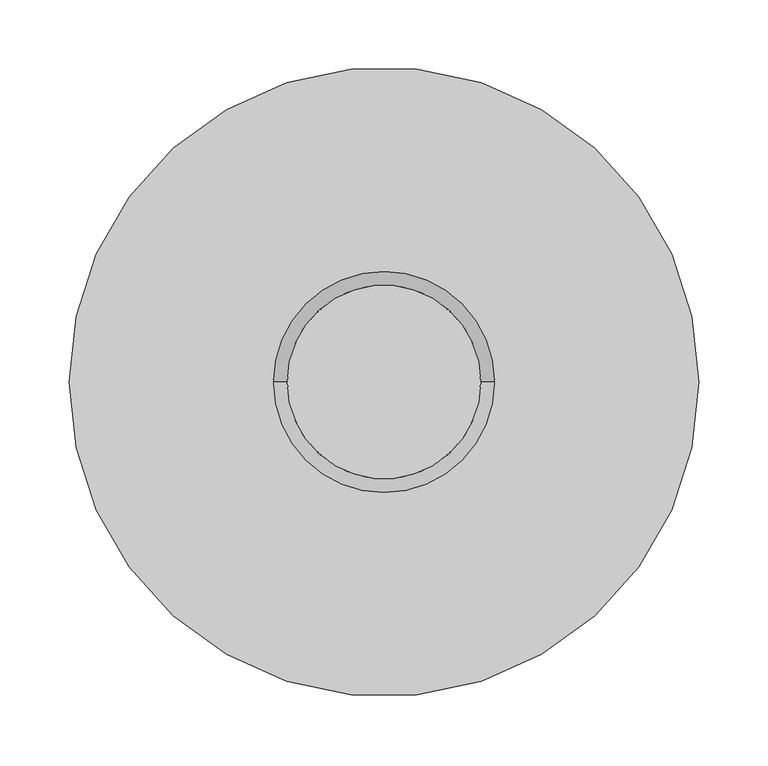
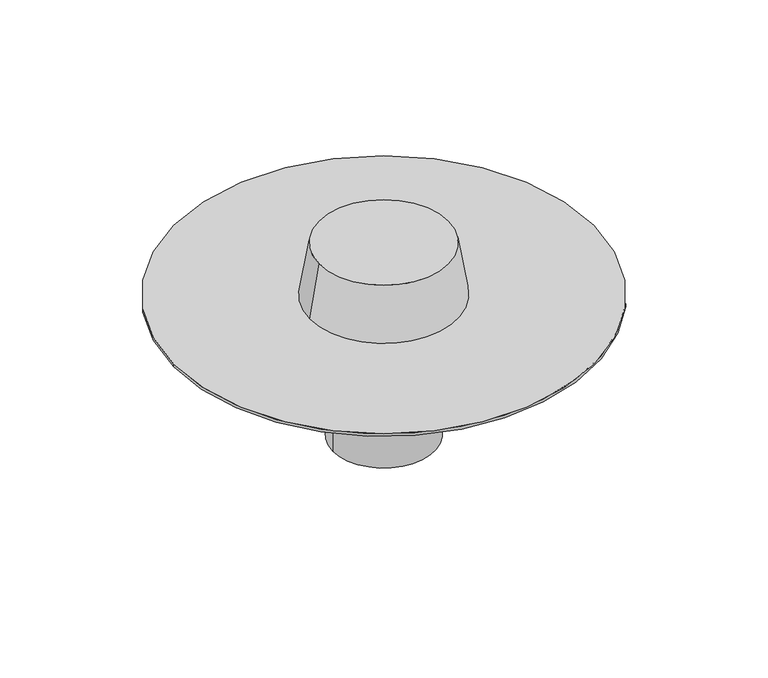
"""IFC4 building model written with IfcOpenShell, lengths in millimetres: proxy geometry, TN_Воронка ТехноНИКОЛЬ ВБ : ВоронкаТехноНИКОЛЬ ВБ, 110х160."""

import ifcopenshell
import ifcopenshell.guid

model = None  # the IFC model being written
_history = None  # IfcOwnerHistory: only IFC2X3 demands one
_inside = {}  # id of a spatial element -> (the spatial element, [elements in it])
_under = {}  # id of a project, library or spatial element -> (it, [spatial elements below it])
_declared = {}  # id of a project -> (the project, [libraries it declares])
_typed = {}  # id of a type object -> (the type object, [elements of that type])
_made_of = {}  # id of a material, layer set ... -> (it, [elements and type objects made of it])


def new_model(schema):
    """Start an empty IFC model of exactly this schema.

    Asked for "IFC4X3", IfcOpenShell would pick the latest addendum, in which some entities
    have other attributes; the version numbers below select the first issue.
    IFC2X3 requires an IfcOwnerHistory on every rooted entity: one is made here for all.
    """
    global model, _history
    if schema == "IFC4X3":
        model = ifcopenshell.file(schema_version=(4, 3, 0, 0))
    else:
        model = ifcopenshell.file(schema=schema)
    _inside.clear()
    _under.clear()
    _declared.clear()
    _typed.clear()
    _made_of.clear()
    _history = None
    if model.schema == "IFC2X3":
        org = make("IfcOrganization", Name="unknown")
        user = make(
            "IfcPersonAndOrganization",
            ThePerson=make("IfcPerson", FamilyName="unknown"),
            TheOrganization=org,
        )
        app = make(
            "IfcApplication",
            ApplicationDeveloper=org,
            Version="unknown",
            ApplicationFullName="unknown",
            ApplicationIdentifier="unknown",
        )
        _history = make(
            "IfcOwnerHistory",
            OwningUser=user,
            OwningApplication=app,
            ChangeAction="ADDED",
            CreationDate=0,
        )
    return model


def make(cls, **values):
    """One entity of the class cls with the attributes given. An attribute that is None is left unset."""
    return model.create_entity(
        cls, **{name: value for name, value in values.items() if value is not None}
    )


def rooted(cls, **values):
    """An entity with a GlobalId (a new one), such as an element, a storey or a relation."""
    return make(cls, GlobalId=ifcopenshell.guid.new(), OwnerHistory=_history, **values)


def si_unit(unit_type, name, prefix=None):
    """IfcSIUnit, for example si_unit("LENGTHUNIT", "METRE", prefix="MILLI")."""
    return make("IfcSIUnit", UnitType=unit_type, Prefix=prefix, Name=name)


def assignment(units):
    """IfcUnitAssignment: the units of a project."""
    return None if units is None else make("IfcUnitAssignment", Units=units)


def point(xyz):
    """IfcCartesianPoint."""
    return None if xyz is None else make("IfcCartesianPoint", Coordinates=xyz)


def direction(xyz):
    """IfcDirection."""
    return None if xyz is None else make("IfcDirection", DirectionRatios=xyz)


def frame(location, z_axis=None, x_axis=None):
    """IfcAxis2Placement3D, a coordinate frame: its origin and axes. An axis left out is left unset."""
    return make(
        "IfcAxis2Placement3D",
        Location=point(location),
        Axis=direction(z_axis),
        RefDirection=direction(x_axis),
    )


def frame_2d(location, x_axis=None):
    """IfcAxis2Placement2D, a coordinate frame in the plane: its origin and x axis."""
    return make(
        "IfcAxis2Placement2D", Location=point(location), RefDirection=direction(x_axis)
    )


def origin():
    """The frame at (0, 0, 0) with its axes left unset."""
    return frame((0.0, 0.0, 0.0))


def origin_2d():
    """The frame at (0, 0) in the plane with its x axis left unset."""
    return frame_2d((0.0, 0.0))


def place(relative_to, where):
    """IfcLocalPlacement: puts the frame where relative to a parent placement (None: the world)."""
    return make(
        "IfcLocalPlacement", PlacementRelTo=relative_to, RelativePlacement=where
    )


def context(
    kind, dimensions, precision=None, world=None, true_north=None, identifier=None
):
    """IfcGeometricRepresentationContext, for example the 3D "Model" context."""
    return make(
        "IfcGeometricRepresentationContext",
        ContextIdentifier=identifier,
        ContextType=kind,
        CoordinateSpaceDimension=dimensions,
        Precision=precision,
        WorldCoordinateSystem=world,
        TrueNorth=true_north,
    )


def project(units=None, contexts=None):
    """IfcProject with its units and contexts."""
    return rooted(
        "IfcProject",
        Name="project",
        RepresentationContexts=contexts,
        UnitsInContext=assignment(units),
    )


def spatial(cls, under=None, at=None, **own):
    """A site, building, storey or space (cls), placed at a placement, below another one or the project."""
    s = rooted(cls, ObjectPlacement=at, **own)
    if under is not None:
        _under.setdefault(under.id(), (under, []))[1].append(s)
    return s


def polyline(points):
    """IfcPolyline through the points."""
    return make("IfcPolyline", Points=[point(p) for p in points])


def circle_curve(where, radius):
    """IfcCircle in the frame where."""
    return make("IfcCircle", Position=where, Radius=radius)


def trimmed(basis, trim1, trim2, sense, master):
    """IfcTrimmedCurve: the piece of a basis curve between two trims."""
    return make(
        "IfcTrimmedCurve",
        BasisCurve=basis,
        Trim1=trim1,
        Trim2=trim2,
        SenseAgreement=sense,
        MasterRepresentation=master,
    )


def segment(curve, same_sense, transition):
    """IfcCompositeCurveSegment."""
    return make(
        "IfcCompositeCurveSegment",
        Transition=transition,
        SameSense=same_sense,
        ParentCurve=curve,
    )


def composite_curve(segments, self_intersect=None):
    """IfcCompositeCurve: segments joined end to end."""
    return make("IfcCompositeCurve", Segments=segments, SelfIntersect=self_intersect)


def outline(outer, holes=None, kind="AREA"):
    """IfcArbitraryClosedProfileDef: a profile drawn as a closed curve; with holes, ...WithVoids."""
    if holes is None:
        return make("IfcArbitraryClosedProfileDef", ProfileType=kind, OuterCurve=outer)
    return make(
        "IfcArbitraryProfileDefWithVoids",
        ProfileType=kind,
        OuterCurve=outer,
        InnerCurves=holes,
    )


def extrude(swept, where, along, depth):
    """IfcExtrudedAreaSolid: the profile swept, set in the frame where, extruded along a direction by depth."""
    return make(
        "IfcExtrudedAreaSolid",
        SweptArea=swept,
        Position=where,
        ExtrudedDirection=direction(along),
        Depth=depth,
    )


def shape(context_of_items, identifier, shape_type, items):
    """IfcShapeRepresentation: the items that make up one representation, for example the "Body"."""
    return make(
        "IfcShapeRepresentation",
        ContextOfItems=context_of_items,
        RepresentationIdentifier=identifier,
        RepresentationType=shape_type,
        Items=items,
    )


def source(mapping_origin, context_of_items, identifier, shape_type, items):
    """IfcRepresentationMap: a shape defined once, which mapped items show again and again."""
    return make(
        "IfcRepresentationMap",
        MappingOrigin=mapping_origin,
        MappedRepresentation=shape(context_of_items, identifier, shape_type, items),
    )


def transform(
    local_origin,
    x_axis=None,
    y_axis=None,
    z_axis=None,
    scale=None,
    scale2=None,
    scale3=None,
    uniform=True,
):
    """IfcCartesianTransformationOperator3D, or its non-uniform kind. x_axis, y_axis, z_axis: its Axis1, 2, 3."""
    if uniform:
        return make(
            "IfcCartesianTransformationOperator3D",
            Axis1=direction(x_axis),
            Axis2=direction(y_axis),
            LocalOrigin=point(local_origin),
            Scale=scale,
            Axis3=direction(z_axis),
        )
    return make(
        "IfcCartesianTransformationOperator3DnonUniform",
        Axis1=direction(x_axis),
        Axis2=direction(y_axis),
        LocalOrigin=point(local_origin),
        Scale=scale,
        Axis3=direction(z_axis),
        Scale2=scale2,
        Scale3=scale3,
    )


def mapped(mapping_source, mapping_target):
    """IfcMappedItem: shows the shape of a source again, moved by a transform."""
    return make(
        "IfcMappedItem", MappingSource=mapping_source, MappingTarget=mapping_target
    )


def made_of(thing, what):
    """Note that an element or type object is made of a material, layer set ...; save() writes the relation."""
    if what is not None:
        _made_of.setdefault(what.id(), (what, []))[1].append(thing)
    return thing


def element(
    cls,
    number,
    at=None,
    inside=None,
    cuts=None,
    type_object=None,
    material=None,
    context=None,
    identifier="Body",
    shape_type=None,
    held_by="IfcProductDefinitionShape",
    body=None,
    shapes=None,
    **own,
):
    """One element of the class cls, such as IfcWall. Its Tag is "e" and its number.

    at: its placement. inside: the storey or other place that contains it. cuts: it is an
    opening in that element (IfcRelVoidsElement). A single representation is given by context,
    identifier, shape_type and body (its items); several are given by shapes. held_by: the class
    of the entity that holds the representations. save() writes the other relations.
    """
    e = rooted(cls, Tag="e%d" % number, ObjectPlacement=at, **own)
    if body is not None:
        shapes = [shape(context, identifier, shape_type, body)]
    if shapes is not None:
        e.Representation = make(held_by, Representations=shapes)
    if inside is not None:
        _inside.setdefault(inside.id(), (inside, []))[1].append(e)
    if cuts is not None:
        rooted(
            "IfcRelVoidsElement", RelatingBuildingElement=cuts, RelatedOpeningElement=e
        )
    if type_object is not None:
        _typed.setdefault(type_object.id(), (type_object, []))[1].append(e)
    return made_of(e, material)


def aggregate(whole, parts):
    """IfcRelAggregates: a whole, such as a stair, and the parts it consists of."""
    return rooted("IfcRelAggregates", RelatingObject=whole, RelatedObjects=parts)


def save(model, path):
    """Write the relations noted so far, then the file.

    IfcRelAggregates (storeys below a building ...), IfcRelContainedInSpatialStructure (elements
    in a storey), IfcRelDefinesByType, IfcRelAssociatesMaterial and IfcRelDeclares: one each for
    every whole, place, type object, material and project.
    """
    for whole, parts in _under.values():
        aggregate(whole, parts)
    for where, things in _inside.values():
        rooted(
            "IfcRelContainedInSpatialStructure",
            RelatedElements=things,
            RelatingStructure=where,
        )
    for kind, things in _typed.values():
        rooted("IfcRelDefinesByType", RelatedObjects=things, RelatingType=kind)
    for what, things in _made_of.values():
        rooted("IfcRelAssociatesMaterial", RelatedObjects=things, RelatingMaterial=what)
    for by, libraries in _declared.values():
        rooted("IfcRelDeclares", RelatingContext=by, RelatedDefinitions=libraries)
    model.write(path)


def plane_surface(at):
    """IfcPlane: the flat surface through the origin of the frame at, square to its z axis."""
    return make("IfcPlane", Position=at)


def revolved_surface(curve, axis_point, axis_direction):
    """IfcSurfaceOfRevolution: the curve turned about the line through axis_point along axis_direction."""
    return make(
        "IfcSurfaceOfRevolution",
        SweptCurve=make("IfcArbitraryOpenProfileDef", ProfileType="CURVE", Curve=curve),
        AxisPosition=make("IfcAxis1Placement", Location=point(axis_point), Axis=direction(axis_direction)),
    )


def advanced_brep(points, edges, surfaces, faces):
    """IfcAdvancedBrep: a solid bounded by faces that lie on surfaces and meet in shared edges.

    An edge is (start, end): straight between two places in points (the first is 0);
    or (start, end, curve); or (start, end, curve, False) where it runs against its curve.
    A face is (place in surfaces, loops), or (place, loops, False) where it looks against
    its surface's normal. A loop lists edges by number (the first is 1), with a minus sign
    where the edge is run from its end to its start. The first loop is the outer one.
    """
    corners = [point(p) for p in points]
    vertices = [make("IfcVertexPoint", VertexGeometry=c) for c in corners]
    made = []
    for start, end, *more in edges:
        made.append(
            make(
                "IfcEdgeCurve",
                EdgeStart=vertices[start],
                EdgeEnd=vertices[end],
                EdgeGeometry=more[0] if more else make("IfcPolyline", Points=[corners[start], corners[end]]),
                SameSense=more[1] if len(more) > 1 else True,
            )
        )
    hull = []
    for where, loops, *sense in faces:
        bounds = []
        for j, loop in enumerate(loops):
            ring = [make("IfcOrientedEdge", EdgeElement=made[abs(k) - 1], Orientation=k > 0) for k in loop]
            bounds.append(
                make(
                    "IfcFaceOuterBound" if j == 0 else "IfcFaceBound",
                    Bound=make("IfcEdgeLoop", EdgeList=ring),
                    Orientation=True,
                )
            )
        hull.append(make("IfcAdvancedFace", Bounds=bounds, FaceSurface=surfaces[where], SameSense=sense[0] if sense else True))
    return make("IfcAdvancedBrep", Outer=make("IfcClosedShell", CfsFaces=hull))


def specialty_equipment_725ca240(model_context):
    return source(origin(), model_context, "Body", "SolidModel", [
        advanced_brep(
        [(70.0, 0.0, -85.0), (-70.0, 0.0, -85.0), (55.0, 0.0, -120.0), (-55.0, 0.0, -120.0)],
        [
            (0, 1, circle_curve(frame((0.0, 0.0, -85.0), z_axis=(0.0, 0.0, 1.0), x_axis=(1.0, 0.0, 0.0)), 70.0)),
            (1, 0, circle_curve(frame((0.0, 0.0, -85.0), z_axis=(0.0, 0.0, 1.0), x_axis=(-1.0, 0.0, 0.0)), 70.0)),
            (2, 3, circle_curve(frame((0.0, 0.0, -120.0), z_axis=(0.0, 0.0, -1.0), x_axis=(-1.0, 0.0, 0.0)), 55.0)),
            (3, 2, circle_curve(frame((0.0, 0.0, -120.0), z_axis=(0.0, 0.0, -1.0), x_axis=(1.0, 0.0, 0.0)), 55.0)),
            (3, 1),
            (0, 2),
        ],
        [
            plane_surface(frame((0.0, 0.0, -85.0), z_axis=(0.0, 0.0, 1.0), x_axis=(0.0, 1.0, 0.0))),
            plane_surface(frame((0.0, 0.0, -120.0), z_axis=(0.0, 0.0, -1.0), x_axis=(0.0, 1.0, 0.0))),
            revolved_surface(polyline([(-54.999999996938776, 0.0, -120.0), (-70.0, 0.0, -85.0)]), (0.0, 0.0, -248.3333333), (0.0, 0.0, 1.0)),
            revolved_surface(polyline([(54.999999996938776, 0.0, -120.0), (70.0, 0.0, -85.0)]), (0.0, 0.0, -248.3333333), (0.0, 0.0, 1.0)),
        ],
        [
            (0, [[1, 2]]),
            (1, [[3, 4]]),
            (2, [[-4, 5, -1, 6]]),
            (3, [[-3, -6, -2, -5]]),
        ],
    ),
        extrude(outline(composite_curve([segment(trimmed(circle_curve(origin_2d(), 70.0), [point((-70.0, 0.0))], [point((70.0, 0.0))], False, "CARTESIAN"), True, "CONTINUOUS"), segment(trimmed(circle_curve(origin_2d(), 70.0), [point((70.0, 0.0))], [point((-70.0, 0.0))], False, "CARTESIAN"), True, "CONTINUOUS")], self_intersect=False)), frame((0.0, 0.0, -85.0), z_axis=(0.0, 0.0, 1.0), x_axis=(1.0, 0.0, 0.0)), (0.0, 0.0, 1.0), 82.0),
        extrude(outline(composite_curve([segment(trimmed(circle_curve(origin_2d(), 55.0), [point((55.0, 0.0))], [point((-55.0, 0.0))], False, "CARTESIAN"), True, "CONTINUOUS"), segment(trimmed(circle_curve(origin_2d(), 55.0), [point((-55.0, 0.0))], [point((55.0, 0.0))], False, "CARTESIAN"), True, "CONTINUOUS")], self_intersect=False)), frame((0.0, 0.0, -160.0), z_axis=(0.0, 0.0, 1.0), x_axis=(1.0, 0.0, 0.0)), (0.0, 0.0, 1.0), 40.0),
        extrude(outline(composite_curve([segment(trimmed(circle_curve(origin_2d(), 227.5), [point((-227.5, 0.0))], [point((227.5, 0.0))], False, "CARTESIAN"), True, "CONTINUOUS"), segment(trimmed(circle_curve(origin_2d(), 227.5), [point((227.5, 0.0))], [point((-227.5, 0.0))], False, "CARTESIAN"), True, "CONTINUOUS")], self_intersect=False)), frame((0.0, 0.0, -3.0), z_axis=(0.0, 0.0, 1.0), x_axis=(1.0, 0.0, 0.0)), (0.0, 0.0, 1.0), 3.0),
        advanced_brep(
        [(-70.0, 0.0, 60.0), (70.0, 0.0, 60.0), (-80.0, 0.0, 0.0), (80.0, 0.0, 0.0)],
        [
            (0, 1, circle_curve(frame((0.0, 0.0, 60.0), z_axis=(0.0, 0.0, 1.0), x_axis=(-1.0, 0.0, 0.0)), 70.0)),
            (1, 0, circle_curve(frame((0.0, 0.0, 60.0), z_axis=(0.0, 0.0, 1.0), x_axis=(1.0, 0.0, 0.0)), 70.0)),
            (2, 3, circle_curve(frame((0.0, 0.0, 0.0), z_axis=(0.0, 0.0, -1.0), x_axis=(1.0, 0.0, 0.0)), 80.0)),
            (3, 2, circle_curve(frame((0.0, 0.0, 0.0), z_axis=(0.0, 0.0, -1.0), x_axis=(-1.0, 0.0, 0.0)), 80.0)),
            (3, 1),
            (0, 2),
        ],
        [
            plane_surface(frame((0.0, 0.0, 60.0), z_axis=(0.0, 0.0, 1.0), x_axis=(0.0, -1.0, 0.0))),
            plane_surface(frame((0.0, 0.0, 0.0), z_axis=(0.0, 0.0, -1.0), x_axis=(0.0, -1.0, 0.0))),
            revolved_surface(polyline([(-70.0, 0.0, 60.0), (-80.0, 0.0, 0.0)]), (0.0, 0.0, 480.0), (0.0, 0.0, -1.0)),
            revolved_surface(polyline([(70.0, 0.0, 60.0), (80.0, 0.0, 0.0)]), (0.0, 0.0, 480.0), (0.0, 0.0, -1.0)),
        ],
        [
            (0, [[1, 2]]),
            (1, [[3, 4]]),
            (2, [[-4, 5, -1, 6]]),
            (3, [[-3, -6, -2, -5]]),
        ],
    ),
    ])


if __name__ == "__main__":
    model = new_model("IFC4")
    model_context = context("Model", 3, world=origin())
    ifc_project = project(units=[si_unit("LENGTHUNIT", "METRE", prefix="MILLI")], contexts=[model_context])
    site = spatial("IfcSite", under=ifc_project)
    building = spatial("IfcBuilding", under=site)
    placement = place(None, origin())
    specialty_equipment_shape = specialty_equipment_725ca240(model_context)
    element("IfcBuildingElementProxy", 1, Name="TN_Воронка ТехноНИКОЛЬ ВБ : ВоронкаТехноНИКОЛЬ ВБ, 110х160", ObjectType="TN_Воронка ТехноНИКОЛЬ ВБ : ВоронкаТехноНИКОЛЬ ВБ, 110х160", at=placement, inside=building, context=model_context, shape_type="MappedRepresentation", body=[
        mapped(specialty_equipment_shape, transform((0.0, 0.0, 0.0), x_axis=(1.0, 0.0, 0.0), y_axis=(0.0, 1.0, 0.0), z_axis=(0.0, 0.0, 1.0))),
    ])
    save(model, "model.ifc")

# Revit data of these elements
# Type "TN_Воронка ТехноНИКОЛЬ ВБ : ВоронкаТехноНИКОЛЬ ВБ, 110х160"
#   ADSK_Группирование = "Комплектующие и воронки"
#   Description = "Воронка ВБ используется при ремонте и строительстве зданий и сооружений и предназначена для\nудаления дождевой воды с плоских кровель. Применяется в кровлях из битумных и битумно-полимерных\nрулонных и мастичных материалов с внутренним водостоком. Рекомендуется устанавливать одну\nворонку примерно на каждые 250 м2 кровли, но требуется не менее двух водоотводящих систем на\nкровлю ограниченную парапетами. Пропуская способность 7,8 л/сек."
#   Manufacturer = "ТехноНИКОЛЬ"
#   URL = "http://nav.tn.ru/upload/iblock/67f/67f1681bb0d078f2e8af03b9528f2af6.pdf"
#   ADSK_Примечание = ""
#   ADSK_Обозначение = "ТехноНИКОЛЬ"
#   ADSK_Наименование = "Воронка ТехноНИКОЛЬ ВБ, 110х160"
#   ADSK_Марка = ""
#   ADSK_Код изделия = "33052"
#   ADSK_Завод-изготовитель = "ТехноНИКОЛЬ"
#   ADSK_Единица измерения = "шт."
#   ADSK_Группирование = "Комплектующие и воронки"
#   ADSK_URL страницы изделия = "https://shop.tn.ru/voronka-tehnonikol-vb-110h160-mm"
#   ADSK_URL документации изделия = "https://nav.tn.ru/catalog/krovlya/vodostochnaya-sistema/voronka-tekhnonikol-vb-110kh160-110x450/?sphrase_id=105157"
#   Диаметр фланца = 455 mm
#   Высота воронки = 160 mm
#   ADSK_Масса = 0.8
#   ADSK_Количество = 1
#   Материал = TN_ПВХ_Черный
#   Default Elevation = 0
# Element 1 (IfcBuildingElementProxy, "TN_Воронка ТехноНИКОЛЬ ВБ : ВоронкаТехноНИКОЛЬ ВБ, 110х160")
#   Materials on its faces: "TN_ПВХ_Черный"
# Materials
#   "TN_ПВХ_Черный": class "Типовые", colour RGB 48 48 48, transparency 0, Cost = 0
